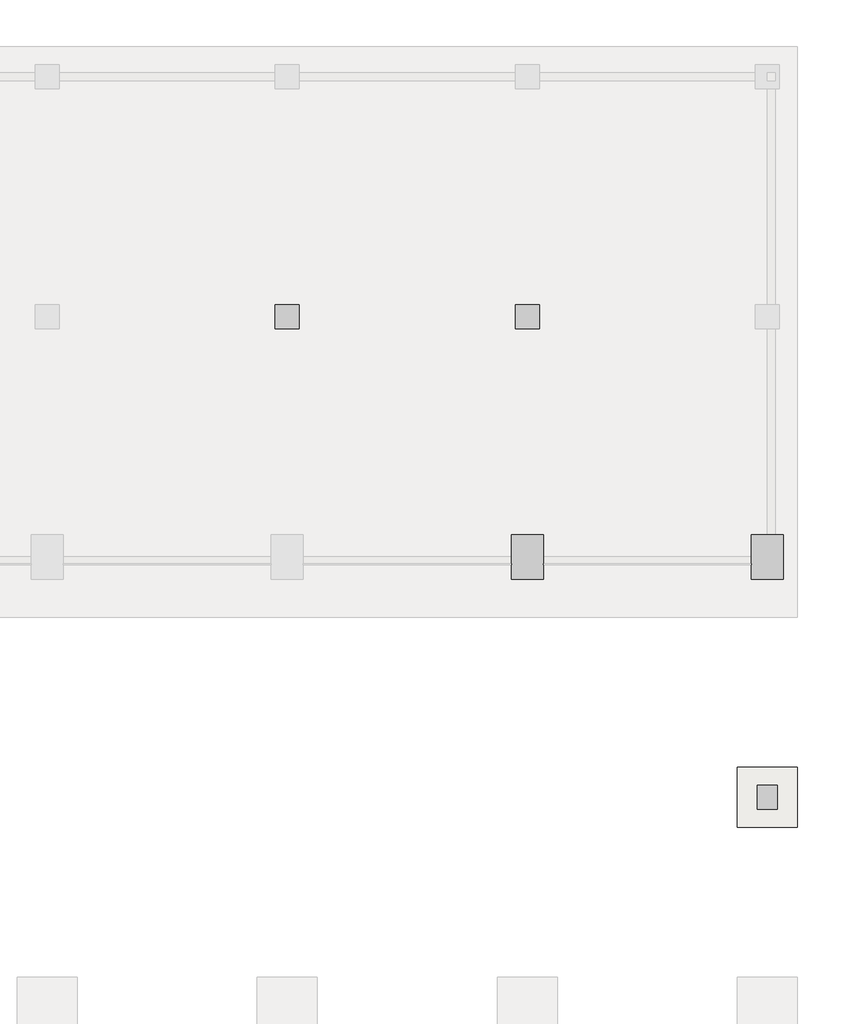
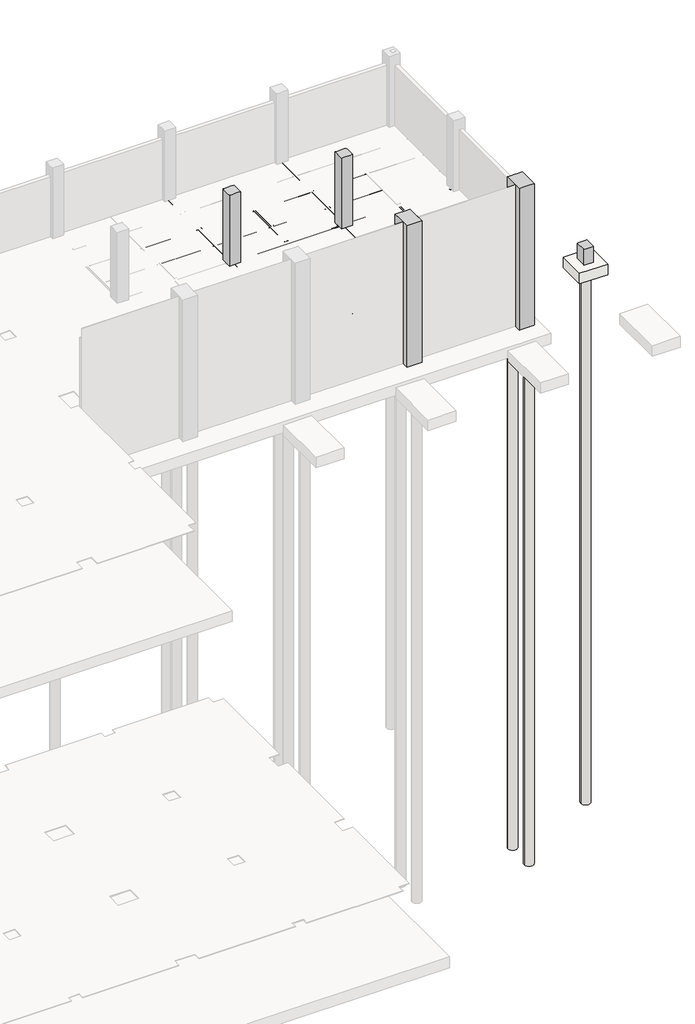
# Not in any storey, part 15 of 16: 29 beams, 5 columns, 4 slabs.
"""IFC4 building model written with IfcOpenShell, lengths in millimetres."""

from ifc_helpers import new_model, si_unit, point, frame, frame_2d, origin, place, context, project, spatial, polyline, circle_curve, trimmed, segment, composite_curve, outline, extrude, faceted_brep, element, save

model = new_model("IFC4")

# Units and contexts
model_context = context("Model", 3, world=origin())
ifc_project = project(units=[si_unit("LENGTHUNIT", "METRE", prefix="MILLI")], contexts=[model_context])

# Site, building
site = spatial("IfcSite", under=ifc_project)
building = spatial("IfcBuilding", under=site)

# Beams
placement = place(None, origin())
element("IfcBeam", 1, ObjectType="Steel Framing_H_KS : H_SB_AR_S02_H-400x200x8x13_BSG2", at=placement, inside=building, context=model_context, shape_type="SweptSolid", body=[
    extrude(outline(composite_curve([segment(polyline([(-4187.0381366, 65900.0), (-4200.0381366, 65900.0), (-4200.0381366, 66100.0), (-4187.0381366, 66100.0), (-4187.0381366, 66020.0)]), True, "CONTINUOUS"), segment(trimmed(circle_curve(frame_2d((-4171.0381366, 66020.0)), 16.0), [point((-4187.0381366, 66020.0))], [point((-4171.0381366, 66004.0))], True, "CARTESIAN"), True, "CONTINUOUS"), segment(polyline([(-4171.0381366, 66004.0), (-3829.0381366, 66004.0)]), True, "CONTINUOUS"), segment(trimmed(circle_curve(frame_2d((-3829.0381366, 66020.0)), 16.0), [point((-3829.0381366, 66004.0))], [point((-3813.0381366, 66020.0))], True, "CARTESIAN"), True, "CONTINUOUS"), segment(polyline([(-3813.0381366, 66020.0), (-3813.0381366, 66100.0), (-3800.0381366, 66100.0), (-3800.0381366, 65900.0), (-3813.0381366, 65900.0), (-3813.0381366, 65980.0)]), True, "CONTINUOUS"), segment(trimmed(circle_curve(frame_2d((-3829.0381366, 65980.0)), 16.0), [point((-3813.0381366, 65980.0))], [point((-3829.0381366, 65996.0))], True, "CARTESIAN"), True, "CONTINUOUS"), segment(polyline([(-3829.0381366, 65996.0), (-4171.0381366, 65996.0)]), True, "CONTINUOUS"), segment(trimmed(circle_curve(frame_2d((-4171.0381366, 65980.0)), 16.0), [point((-4171.0381366, 65996.0))], [point((-4187.0381366, 65980.0))], True, "CARTESIAN"), True, "CONTINUOUS"), segment(polyline([(-4187.0381366, 65980.0), (-4187.0381366, 65900.0)]), True, "CONTINUOUS")], self_intersect=False)), frame((0.0, -11687.3, 0.0), z_axis=(0.0, 1.0, 0.0), x_axis=(0.0, 0.0, 1.0)), (0.0, 0.0, 1.0), 5374.6),
])
element("IfcBeam", 2, ObjectType="Steel Framing_C_KS : H_SB_AR_S02_C-150x75x6.5x10_J1", at=placement, inside=building, context=model_context, shape_type="SweptSolid", body=[
    extrude(outline(composite_curve([segment(polyline([(-8977.2, -3800.0381366), (-8977.2, -3950.0381366), (-9052.2, -3950.0381366)]), True, "CONTINUOUS"), segment(trimmed(circle_curve(frame_2d((-9042.2, -3950.0381366)), 10.0), [point((-9052.2, -3950.0381366))], [point((-9042.2, -3940.0381366))], False, "CARTESIAN"), True, "CONTINUOUS"), segment(polyline([(-9042.2, -3940.0381366), (-8983.7, -3930.7726469), (-8983.7, -3819.3036264), (-9042.2, -3810.0381366)]), True, "CONTINUOUS"), segment(trimmed(circle_curve(frame_2d((-9042.2, -3800.0381366)), 10.0), [point((-9042.2, -3810.0381366))], [point((-9052.2, -3800.0381366))], False, "CARTESIAN"), True, "CONTINUOUS"), segment(polyline([(-9052.2, -3800.0381366), (-8977.2, -3800.0381366)]), True, "CONTINUOUS")], self_intersect=False)), frame((63112.7, 0.0, 0.0), z_axis=(1.0, 0.0, 0.0), x_axis=(0.0, 1.0, 0.0)), (0.0, 0.0, 1.0), 2774.6),
])
element("IfcBeam", 3, ObjectType="Steel Framing_C_KS : H_SB_AR_S02_C-150x75x6.5x10_J1", at=placement, inside=building, context=model_context, shape_type="SweptSolid", body=[
    extrude(outline(composite_curve([segment(polyline([(-10477.2, -3800.0381366), (-10477.2, -3950.0381366), (-10552.2, -3950.0381366)]), True, "CONTINUOUS"), segment(trimmed(circle_curve(frame_2d((-10542.2, -3950.0381366)), 10.0), [point((-10552.2, -3950.0381366))], [point((-10542.2, -3940.0381366))], False, "CARTESIAN"), True, "CONTINUOUS"), segment(polyline([(-10542.2, -3940.0381366), (-10483.7, -3930.7726469), (-10483.7, -3819.3036264), (-10542.2, -3810.0381366)]), True, "CONTINUOUS"), segment(trimmed(circle_curve(frame_2d((-10542.2, -3800.0381366)), 10.0), [point((-10542.2, -3810.0381366))], [point((-10552.2, -3800.0381366))], False, "CARTESIAN"), True, "CONTINUOUS"), segment(polyline([(-10552.2, -3800.0381366), (-10477.2, -3800.0381366)]), True, "CONTINUOUS")], self_intersect=False)), frame((63112.7, 0.0, 0.0), z_axis=(1.0, 0.0, 0.0), x_axis=(0.0, 1.0, 0.0)), (0.0, 0.0, 1.0), 2774.6),
])
element("IfcBeam", 4, ObjectType="Steel Framing_H_KS : H_SB_AR_S02_H-400x200x8x13_BSG1", at=placement, inside=building, context=model_context, shape_type="SweptSolid", body=[
    extrude(outline(composite_curve([segment(polyline([(-11900.0, -4187.0381366), (-11900.0, -4200.0381366), (-12100.0, -4200.0381366), (-12100.0, -4187.0381366), (-12020.0, -4187.0381366)]), True, "CONTINUOUS"), segment(trimmed(circle_curve(frame_2d((-12020.0, -4171.0381366)), 16.0), [point((-12020.0, -4187.0381366))], [point((-12004.0, -4171.0381366))], True, "CARTESIAN"), True, "CONTINUOUS"), segment(polyline([(-12004.0, -4171.0381366), (-12004.0, -3829.0381366)]), True, "CONTINUOUS"), segment(trimmed(circle_curve(frame_2d((-12020.0, -3829.0381366)), 16.0), [point((-12004.0, -3829.0381366))], [point((-12020.0, -3813.0381366))], True, "CARTESIAN"), True, "CONTINUOUS"), segment(polyline([(-12020.0, -3813.0381366), (-12100.0, -3813.0381366), (-12100.0, -3800.0381366), (-11900.0, -3800.0381366), (-11900.0, -3813.0381366), (-11980.0, -3813.0381366)]), True, "CONTINUOUS"), segment(trimmed(circle_curve(frame_2d((-11980.0, -3829.0381366)), 16.0), [point((-11980.0, -3813.0381366))], [point((-11996.0, -3829.0381366))], True, "CARTESIAN"), True, "CONTINUOUS"), segment(polyline([(-11996.0, -3829.0381366), (-11996.0, -4171.0381366)]), True, "CONTINUOUS"), segment(trimmed(circle_curve(frame_2d((-11980.0, -4171.0381366)), 16.0), [point((-11996.0, -4171.0381366))], [point((-11980.0, -4187.0381366))], True, "CARTESIAN"), True, "CONTINUOUS"), segment(polyline([(-11980.0, -4187.0381366), (-11900.0, -4187.0381366)]), True, "CONTINUOUS")], self_intersect=False)), frame((66312.7, 0.0, 0.0), z_axis=(1.0, 0.0, 0.0), x_axis=(0.0, 1.0, 0.0)), (0.0, 0.0, 1.0), 5374.6),
])
element("IfcBeam", 5, ObjectType="Steel Framing_H_KS : H_SB_AR_S02_H-400x200x8x13_BSG2", at=placement, inside=building, context=model_context, shape_type="SweptSolid", body=[
    extrude(outline(composite_curve([segment(polyline([(-4187.0381366, 71900.0), (-4200.0381366, 71900.0), (-4200.0381366, 72100.0), (-4187.0381366, 72100.0), (-4187.0381366, 72020.0)]), True, "CONTINUOUS"), segment(trimmed(circle_curve(frame_2d((-4171.0381366, 72020.0)), 16.0), [point((-4187.0381366, 72020.0))], [point((-4171.0381366, 72004.0))], True, "CARTESIAN"), True, "CONTINUOUS"), segment(polyline([(-4171.0381366, 72004.0), (-3829.0381366, 72004.0)]), True, "CONTINUOUS"), segment(trimmed(circle_curve(frame_2d((-3829.0381366, 72020.0)), 16.0), [point((-3829.0381366, 72004.0))], [point((-3813.0381366, 72020.0))], True, "CARTESIAN"), True, "CONTINUOUS"), segment(polyline([(-3813.0381366, 72020.0), (-3813.0381366, 72100.0), (-3800.0381366, 72100.0), (-3800.0381366, 71900.0), (-3813.0381366, 71900.0), (-3813.0381366, 71980.0)]), True, "CONTINUOUS"), segment(trimmed(circle_curve(frame_2d((-3829.0381366, 71980.0)), 16.0), [point((-3813.0381366, 71980.0))], [point((-3829.0381366, 71996.0))], True, "CARTESIAN"), True, "CONTINUOUS"), segment(polyline([(-3829.0381366, 71996.0), (-4171.0381366, 71996.0)]), True, "CONTINUOUS"), segment(trimmed(circle_curve(frame_2d((-4171.0381366, 71980.0)), 16.0), [point((-4171.0381366, 71996.0))], [point((-4187.0381366, 71980.0))], True, "CARTESIAN"), True, "CONTINUOUS"), segment(polyline([(-4187.0381366, 71980.0), (-4187.0381366, 71900.0)]), True, "CONTINUOUS")], self_intersect=False)), frame((0.0, -11687.3, 0.0), z_axis=(0.0, 1.0, 0.0), x_axis=(0.0, 0.0, 1.0)), (0.0, 0.0, 1.0), 5374.6),
])
element("IfcBeam", 6, ObjectType="Steel Framing_H_KS : H_SB_AR_S02_H-400x200x8x13_BSB1", at=placement, inside=building, context=model_context, shape_type="SweptSolid", body=[
    extrude(outline(composite_curve([segment(polyline([(-4187.0381366, 68900.0), (-4200.0381366, 68900.0), (-4200.0381366, 69100.0), (-4187.0381366, 69100.0), (-4187.0381366, 69020.0)]), True, "CONTINUOUS"), segment(trimmed(circle_curve(frame_2d((-4171.0381366, 69020.0)), 16.0), [point((-4187.0381366, 69020.0))], [point((-4171.0381366, 69004.0))], True, "CARTESIAN"), True, "CONTINUOUS"), segment(polyline([(-4171.0381366, 69004.0), (-3829.0381366, 69004.0)]), True, "CONTINUOUS"), segment(trimmed(circle_curve(frame_2d((-3829.0381366, 69020.0)), 16.0), [point((-3829.0381366, 69004.0))], [point((-3813.0381366, 69020.0))], True, "CARTESIAN"), True, "CONTINUOUS"), segment(polyline([(-3813.0381366, 69020.0), (-3813.0381366, 69100.0), (-3800.0381366, 69100.0), (-3800.0381366, 68900.0), (-3813.0381366, 68900.0), (-3813.0381366, 68980.0)]), True, "CONTINUOUS"), segment(trimmed(circle_curve(frame_2d((-3829.0381366, 68980.0)), 16.0), [point((-3813.0381366, 68980.0))], [point((-3829.0381366, 68996.0))], True, "CARTESIAN"), True, "CONTINUOUS"), segment(polyline([(-3829.0381366, 68996.0), (-4171.0381366, 68996.0)]), True, "CONTINUOUS"), segment(trimmed(circle_curve(frame_2d((-4171.0381366, 68980.0)), 16.0), [point((-4171.0381366, 68996.0))], [point((-4187.0381366, 68980.0))], True, "CARTESIAN"), True, "CONTINUOUS"), segment(polyline([(-4187.0381366, 68980.0), (-4187.0381366, 68900.0)]), True, "CONTINUOUS")], self_intersect=False)), frame((0.0, -11887.3, 0.0), z_axis=(0.0, 1.0, 0.0), x_axis=(0.0, 0.0, 1.0)), (0.0, 0.0, 1.0), 5887.3),
])
element("IfcBeam", 7, ObjectType="Steel Framing_C_KS : H_SB_AR_S02_C-150x75x6.5x10_J1", at=placement, inside=building, context=model_context, shape_type="SweptSolid", body=[
    extrude(outline(composite_curve([segment(polyline([(-8977.2, -3800.0381366), (-8977.2, -3950.0381366), (-9052.2, -3950.0381366)]), True, "CONTINUOUS"), segment(trimmed(circle_curve(frame_2d((-9042.2, -3950.0381366)), 10.0), [point((-9052.2, -3950.0381366))], [point((-9042.2, -3940.0381366))], False, "CARTESIAN"), True, "CONTINUOUS"), segment(polyline([(-9042.2, -3940.0381366), (-8983.7, -3930.7726469), (-8983.7, -3819.3036264), (-9042.2, -3810.0381366)]), True, "CONTINUOUS"), segment(trimmed(circle_curve(frame_2d((-9042.2, -3800.0381366)), 10.0), [point((-9042.2, -3810.0381366))], [point((-9052.2, -3800.0381366))], False, "CARTESIAN"), True, "CONTINUOUS"), segment(polyline([(-9052.2, -3800.0381366), (-8977.2, -3800.0381366)]), True, "CONTINUOUS")], self_intersect=False)), frame((66112.7, 0.0, 0.0), z_axis=(1.0, 0.0, 0.0), x_axis=(0.0, 1.0, 0.0)), (0.0, 0.0, 1.0), 2774.6),
])
element("IfcBeam", 8, ObjectType="Steel Framing_C_KS : H_SB_AR_S02_C-150x75x6.5x10_J1", at=placement, inside=building, context=model_context, shape_type="SweptSolid", body=[
    extrude(outline(composite_curve([segment(polyline([(-10477.2, -3800.0381366), (-10477.2, -3950.0381366), (-10552.2, -3950.0381366)]), True, "CONTINUOUS"), segment(trimmed(circle_curve(frame_2d((-10542.2, -3950.0381366)), 10.0), [point((-10552.2, -3950.0381366))], [point((-10542.2, -3940.0381366))], False, "CARTESIAN"), True, "CONTINUOUS"), segment(polyline([(-10542.2, -3940.0381366), (-10483.7, -3930.7726469), (-10483.7, -3819.3036264), (-10542.2, -3810.0381366)]), True, "CONTINUOUS"), segment(trimmed(circle_curve(frame_2d((-10542.2, -3800.0381366)), 10.0), [point((-10542.2, -3810.0381366))], [point((-10552.2, -3800.0381366))], False, "CARTESIAN"), True, "CONTINUOUS"), segment(polyline([(-10552.2, -3800.0381366), (-10477.2, -3800.0381366)]), True, "CONTINUOUS")], self_intersect=False)), frame((66112.7, 0.0, 0.0), z_axis=(1.0, 0.0, 0.0), x_axis=(0.0, 1.0, 0.0)), (0.0, 0.0, 1.0), 2774.6),
])
element("IfcBeam", 9, ObjectType="Steel Framing_C_KS : H_SB_AR_S02_C-150x75x6.5x10_J1", at=placement, inside=building, context=model_context, shape_type="SweptSolid", body=[
    extrude(outline(composite_curve([segment(polyline([(-8977.2, -3800.0381366), (-8977.2, -3950.0381366), (-9052.2, -3950.0381366)]), True, "CONTINUOUS"), segment(trimmed(circle_curve(frame_2d((-9042.2, -3950.0381366)), 10.0), [point((-9052.2, -3950.0381366))], [point((-9042.2, -3940.0381366))], False, "CARTESIAN"), True, "CONTINUOUS"), segment(polyline([(-9042.2, -3940.0381366), (-8983.7, -3930.7726469), (-8983.7, -3819.3036264), (-9042.2, -3810.0381366)]), True, "CONTINUOUS"), segment(trimmed(circle_curve(frame_2d((-9042.2, -3800.0381366)), 10.0), [point((-9042.2, -3810.0381366))], [point((-9052.2, -3800.0381366))], False, "CARTESIAN"), True, "CONTINUOUS"), segment(polyline([(-9052.2, -3800.0381366), (-8977.2, -3800.0381366)]), True, "CONTINUOUS")], self_intersect=False)), frame((69112.7, 0.0, 0.0), z_axis=(1.0, 0.0, 0.0), x_axis=(0.0, 1.0, 0.0)), (0.0, 0.0, 1.0), 2774.6),
])
element("IfcBeam", 10, ObjectType="Steel Framing_C_KS : H_SB_AR_S02_C-150x75x6.5x10_J1", at=placement, inside=building, context=model_context, shape_type="SweptSolid", body=[
    extrude(outline(composite_curve([segment(polyline([(-10477.2, -3800.0381366), (-10477.2, -3950.0381366), (-10552.2, -3950.0381366)]), True, "CONTINUOUS"), segment(trimmed(circle_curve(frame_2d((-10542.2, -3950.0381366)), 10.0), [point((-10552.2, -3950.0381366))], [point((-10542.2, -3940.0381366))], False, "CARTESIAN"), True, "CONTINUOUS"), segment(polyline([(-10542.2, -3940.0381366), (-10483.7, -3930.7726469), (-10483.7, -3819.3036264), (-10542.2, -3810.0381366)]), True, "CONTINUOUS"), segment(trimmed(circle_curve(frame_2d((-10542.2, -3800.0381366)), 10.0), [point((-10542.2, -3810.0381366))], [point((-10552.2, -3800.0381366))], False, "CARTESIAN"), True, "CONTINUOUS"), segment(polyline([(-10552.2, -3800.0381366), (-10477.2, -3800.0381366)]), True, "CONTINUOUS")], self_intersect=False)), frame((69112.7, 0.0, 0.0), z_axis=(1.0, 0.0, 0.0), x_axis=(0.0, 1.0, 0.0)), (0.0, 0.0, 1.0), 2774.6),
])
element("IfcBeam", 11, ObjectType="Steel Framing_H_KS : H_SB_AR_S02_H-400x200x8x13_BSG1", at=placement, inside=building, context=model_context, shape_type="SweptSolid", body=[
    extrude(outline(composite_curve([segment(polyline([(-11900.0, -4187.0381366), (-11900.0, -4200.0381366), (-12100.0, -4200.0381366), (-12100.0, -4187.0381366), (-12020.0, -4187.0381366)]), True, "CONTINUOUS"), segment(trimmed(circle_curve(frame_2d((-12020.0, -4171.0381366)), 16.0), [point((-12020.0, -4187.0381366))], [point((-12004.0, -4171.0381366))], True, "CARTESIAN"), True, "CONTINUOUS"), segment(polyline([(-12004.0, -4171.0381366), (-12004.0, -3829.0381366)]), True, "CONTINUOUS"), segment(trimmed(circle_curve(frame_2d((-12020.0, -3829.0381366)), 16.0), [point((-12004.0, -3829.0381366))], [point((-12020.0, -3813.0381366))], True, "CARTESIAN"), True, "CONTINUOUS"), segment(polyline([(-12020.0, -3813.0381366), (-12100.0, -3813.0381366), (-12100.0, -3800.0381366), (-11900.0, -3800.0381366), (-11900.0, -3813.0381366), (-11980.0, -3813.0381366)]), True, "CONTINUOUS"), segment(trimmed(circle_curve(frame_2d((-11980.0, -3829.0381366)), 16.0), [point((-11980.0, -3813.0381366))], [point((-11996.0, -3829.0381366))], True, "CARTESIAN"), True, "CONTINUOUS"), segment(polyline([(-11996.0, -3829.0381366), (-11996.0, -4171.0381366)]), True, "CONTINUOUS"), segment(trimmed(circle_curve(frame_2d((-11980.0, -4171.0381366)), 16.0), [point((-11996.0, -4171.0381366))], [point((-11980.0, -4187.0381366))], True, "CARTESIAN"), True, "CONTINUOUS"), segment(polyline([(-11980.0, -4187.0381366), (-11900.0, -4187.0381366)]), True, "CONTINUOUS")], self_intersect=False)), frame((72312.7, 0.0, 0.0), z_axis=(1.0, 0.0, 0.0), x_axis=(0.0, 1.0, 0.0)), (0.0, 0.0, 1.0), 5374.6),
])
element("IfcBeam", 12, ObjectType="Steel Framing_C_KS : H_SB_AR_S02_C-150x75x6.5x10_J1", at=placement, inside=building, context=model_context, shape_type="SweptSolid", body=[
    extrude(outline(composite_curve([segment(polyline([(-8977.2, -3800.0381366), (-8977.2, -3950.0381366), (-9052.2, -3950.0381366)]), True, "CONTINUOUS"), segment(trimmed(circle_curve(frame_2d((-9042.2, -3950.0381366)), 10.0), [point((-9052.2, -3950.0381366))], [point((-9042.2, -3940.0381366))], False, "CARTESIAN"), True, "CONTINUOUS"), segment(polyline([(-9042.2, -3940.0381366), (-8983.7, -3930.7726469), (-8983.7, -3819.3036264), (-9042.2, -3810.0381366)]), True, "CONTINUOUS"), segment(trimmed(circle_curve(frame_2d((-9042.2, -3800.0381366)), 10.0), [point((-9042.2, -3810.0381366))], [point((-9052.2, -3800.0381366))], False, "CARTESIAN"), True, "CONTINUOUS"), segment(polyline([(-9052.2, -3800.0381366), (-8977.2, -3800.0381366)]), True, "CONTINUOUS")], self_intersect=False)), frame((72112.7, 0.0, 0.0), z_axis=(1.0, 0.0, 0.0), x_axis=(0.0, 1.0, 0.0)), (0.0, 0.0, 1.0), 2774.6),
])
element("IfcBeam", 13, ObjectType="Steel Framing_C_KS : H_SB_AR_S02_C-150x75x6.5x10_J1", at=placement, inside=building, context=model_context, shape_type="SweptSolid", body=[
    extrude(outline(composite_curve([segment(polyline([(-10477.2, -3800.0381366), (-10477.2, -3950.0381366), (-10552.2, -3950.0381366)]), True, "CONTINUOUS"), segment(trimmed(circle_curve(frame_2d((-10542.2, -3950.0381366)), 10.0), [point((-10552.2, -3950.0381366))], [point((-10542.2, -3940.0381366))], False, "CARTESIAN"), True, "CONTINUOUS"), segment(polyline([(-10542.2, -3940.0381366), (-10483.7, -3930.7726469), (-10483.7, -3819.3036264), (-10542.2, -3810.0381366)]), True, "CONTINUOUS"), segment(trimmed(circle_curve(frame_2d((-10542.2, -3800.0381366)), 10.0), [point((-10542.2, -3810.0381366))], [point((-10552.2, -3800.0381366))], False, "CARTESIAN"), True, "CONTINUOUS"), segment(polyline([(-10552.2, -3800.0381366), (-10477.2, -3800.0381366)]), True, "CONTINUOUS")], self_intersect=False)), frame((72112.7, 0.0, 0.0), z_axis=(1.0, 0.0, 0.0), x_axis=(0.0, 1.0, 0.0)), (0.0, 0.0, 1.0), 2774.6),
])
element("IfcBeam", 14, ObjectType="Steel Framing_H_KS : H_SB_AR_S02_H-400x200x8x13_BSG2", at=placement, inside=building, context=model_context, shape_type="SweptSolid", body=[
    extrude(outline(composite_curve([segment(polyline([(-4187.0381366, 65900.0), (-4200.0381366, 65900.0), (-4200.0381366, 66100.0), (-4187.0381366, 66100.0), (-4187.0381366, 66020.0)]), True, "CONTINUOUS"), segment(trimmed(circle_curve(frame_2d((-4171.0381366, 66020.0)), 16.0), [point((-4187.0381366, 66020.0))], [point((-4171.0381366, 66004.0))], True, "CARTESIAN"), True, "CONTINUOUS"), segment(polyline([(-4171.0381366, 66004.0), (-3829.0381366, 66004.0)]), True, "CONTINUOUS"), segment(trimmed(circle_curve(frame_2d((-3829.0381366, 66020.0)), 16.0), [point((-3829.0381366, 66004.0))], [point((-3813.0381366, 66020.0))], True, "CARTESIAN"), True, "CONTINUOUS"), segment(polyline([(-3813.0381366, 66020.0), (-3813.0381366, 66100.0), (-3800.0381366, 66100.0), (-3800.0381366, 65900.0), (-3813.0381366, 65900.0), (-3813.0381366, 65980.0)]), True, "CONTINUOUS"), segment(trimmed(circle_curve(frame_2d((-3829.0381366, 65980.0)), 16.0), [point((-3813.0381366, 65980.0))], [point((-3829.0381366, 65996.0))], True, "CARTESIAN"), True, "CONTINUOUS"), segment(polyline([(-3829.0381366, 65996.0), (-4171.0381366, 65996.0)]), True, "CONTINUOUS"), segment(trimmed(circle_curve(frame_2d((-4171.0381366, 65980.0)), 16.0), [point((-4171.0381366, 65996.0))], [point((-4187.0381366, 65980.0))], True, "CARTESIAN"), True, "CONTINUOUS"), segment(polyline([(-4187.0381366, 65980.0), (-4187.0381366, 65900.0)]), True, "CONTINUOUS")], self_intersect=False)), frame((0.0, -17437.3, 0.0), z_axis=(0.0, 1.0, 0.0), x_axis=(0.0, 0.0, 1.0)), (0.0, 0.0, 1.0), 5124.6),
])
element("IfcBeam", 15, ObjectType="Steel Framing_C_KS : H_SB_AR_S02_C-150x75x6.5x10_J1", at=placement, inside=building, context=model_context, shape_type="SweptSolid", body=[
    extrude(outline(composite_curve([segment(polyline([(-14977.2, -3800.0381366), (-14977.2, -3950.0381366), (-15052.2, -3950.0381366)]), True, "CONTINUOUS"), segment(trimmed(circle_curve(frame_2d((-15042.2, -3950.0381366)), 10.0), [point((-15052.2, -3950.0381366))], [point((-15042.2, -3940.0381366))], False, "CARTESIAN"), True, "CONTINUOUS"), segment(polyline([(-15042.2, -3940.0381366), (-14983.7, -3930.7726469), (-14983.7, -3819.3036264), (-15042.2, -3810.0381366)]), True, "CONTINUOUS"), segment(trimmed(circle_curve(frame_2d((-15042.2, -3800.0381366)), 10.0), [point((-15042.2, -3810.0381366))], [point((-15052.2, -3800.0381366))], False, "CARTESIAN"), True, "CONTINUOUS"), segment(polyline([(-15052.2, -3800.0381366), (-14977.2, -3800.0381366)]), True, "CONTINUOUS")], self_intersect=False)), frame((63112.7, 0.0, 0.0), z_axis=(1.0, 0.0, 0.0), x_axis=(0.0, 1.0, 0.0)), (0.0, 0.0, 1.0), 2774.6),
])
element("IfcBeam", 16, ObjectType="Steel Framing_C_KS : H_SB_AR_S02_C-150x75x6.5x10_J1", at=placement, inside=building, context=model_context, shape_type="SweptSolid", body=[
    extrude(outline(composite_curve([segment(polyline([(-13477.2, -3800.0381366), (-13477.2, -3950.0381366), (-13552.2, -3950.0381366)]), True, "CONTINUOUS"), segment(trimmed(circle_curve(frame_2d((-13542.2, -3950.0381366)), 10.0), [point((-13552.2, -3950.0381366))], [point((-13542.2, -3940.0381366))], False, "CARTESIAN"), True, "CONTINUOUS"), segment(polyline([(-13542.2, -3940.0381366), (-13483.7, -3930.7726469), (-13483.7, -3819.3036264), (-13542.2, -3810.0381366)]), True, "CONTINUOUS"), segment(trimmed(circle_curve(frame_2d((-13542.2, -3800.0381366)), 10.0), [point((-13542.2, -3810.0381366))], [point((-13552.2, -3800.0381366))], False, "CARTESIAN"), True, "CONTINUOUS"), segment(polyline([(-13552.2, -3800.0381366), (-13477.2, -3800.0381366)]), True, "CONTINUOUS")], self_intersect=False)), frame((63112.7, 0.0, 0.0), z_axis=(1.0, 0.0, 0.0), x_axis=(0.0, 1.0, 0.0)), (0.0, 0.0, 1.0), 2774.6),
])
element("IfcBeam", 17, ObjectType="Steel Framing_H_KS : H_SB_AR_S02_H-400x200x8x13_BSG2", at=placement, inside=building, context=model_context, shape_type="SweptSolid", body=[
    extrude(outline(composite_curve([segment(polyline([(-4187.0381366, 71900.0), (-4200.0381366, 71900.0), (-4200.0381366, 72100.0), (-4187.0381366, 72100.0), (-4187.0381366, 72020.0)]), True, "CONTINUOUS"), segment(trimmed(circle_curve(frame_2d((-4171.0381366, 72020.0)), 16.0), [point((-4187.0381366, 72020.0))], [point((-4171.0381366, 72004.0))], True, "CARTESIAN"), True, "CONTINUOUS"), segment(polyline([(-4171.0381366, 72004.0), (-3829.0381366, 72004.0)]), True, "CONTINUOUS"), segment(trimmed(circle_curve(frame_2d((-3829.0381366, 72020.0)), 16.0), [point((-3829.0381366, 72004.0))], [point((-3813.0381366, 72020.0))], True, "CARTESIAN"), True, "CONTINUOUS"), segment(polyline([(-3813.0381366, 72020.0), (-3813.0381366, 72100.0), (-3800.0381366, 72100.0), (-3800.0381366, 71900.0), (-3813.0381366, 71900.0), (-3813.0381366, 71980.0)]), True, "CONTINUOUS"), segment(trimmed(circle_curve(frame_2d((-3829.0381366, 71980.0)), 16.0), [point((-3813.0381366, 71980.0))], [point((-3829.0381366, 71996.0))], True, "CARTESIAN"), True, "CONTINUOUS"), segment(polyline([(-3829.0381366, 71996.0), (-4171.0381366, 71996.0)]), True, "CONTINUOUS"), segment(trimmed(circle_curve(frame_2d((-4171.0381366, 71980.0)), 16.0), [point((-4171.0381366, 71996.0))], [point((-4187.0381366, 71980.0))], True, "CARTESIAN"), True, "CONTINUOUS"), segment(polyline([(-4187.0381366, 71980.0), (-4187.0381366, 71900.0)]), True, "CONTINUOUS")], self_intersect=False)), frame((0.0, -17437.3, 0.0), z_axis=(0.0, 1.0, 0.0), x_axis=(0.0, 0.0, 1.0)), (0.0, 0.0, 1.0), 5124.6),
])
element("IfcBeam", 18, ObjectType="Steel Framing_H_KS : H_SB_AR_S02_H-400x200x8x13_BSB1", at=placement, inside=building, context=model_context, shape_type="SweptSolid", body=[
    extrude(outline(composite_curve([segment(polyline([(-4187.0381366, 68900.0), (-4200.0381366, 68900.0), (-4200.0381366, 69100.0), (-4187.0381366, 69100.0), (-4187.0381366, 69020.0)]), True, "CONTINUOUS"), segment(trimmed(circle_curve(frame_2d((-4171.0381366, 69020.0)), 16.0), [point((-4187.0381366, 69020.0))], [point((-4171.0381366, 69004.0))], True, "CARTESIAN"), True, "CONTINUOUS"), segment(polyline([(-4171.0381366, 69004.0), (-3829.0381366, 69004.0)]), True, "CONTINUOUS"), segment(trimmed(circle_curve(frame_2d((-3829.0381366, 69020.0)), 16.0), [point((-3829.0381366, 69004.0))], [point((-3813.0381366, 69020.0))], True, "CARTESIAN"), True, "CONTINUOUS"), segment(polyline([(-3813.0381366, 69020.0), (-3813.0381366, 69100.0), (-3800.0381366, 69100.0), (-3800.0381366, 68900.0), (-3813.0381366, 68900.0), (-3813.0381366, 68980.0)]), True, "CONTINUOUS"), segment(trimmed(circle_curve(frame_2d((-3829.0381366, 68980.0)), 16.0), [point((-3813.0381366, 68980.0))], [point((-3829.0381366, 68996.0))], True, "CARTESIAN"), True, "CONTINUOUS"), segment(polyline([(-3829.0381366, 68996.0), (-4171.0381366, 68996.0)]), True, "CONTINUOUS"), segment(trimmed(circle_curve(frame_2d((-4171.0381366, 68980.0)), 16.0), [point((-4171.0381366, 68996.0))], [point((-4187.0381366, 68980.0))], True, "CARTESIAN"), True, "CONTINUOUS"), segment(polyline([(-4187.0381366, 68980.0), (-4187.0381366, 68900.0)]), True, "CONTINUOUS")], self_intersect=False)), frame((0.0, -18000.0, 0.0), z_axis=(0.0, 1.0, 0.0), x_axis=(0.0, 0.0, 1.0)), (0.0, 0.0, 1.0), 5887.3),
])
element("IfcBeam", 19, ObjectType="Steel Framing_C_KS : H_SB_AR_S02_C-150x75x6.5x10_J1", at=placement, inside=building, context=model_context, shape_type="SweptSolid", body=[
    extrude(outline(composite_curve([segment(polyline([(-14977.2, -3800.0381366), (-14977.2, -3950.0381366), (-15052.2, -3950.0381366)]), True, "CONTINUOUS"), segment(trimmed(circle_curve(frame_2d((-15042.2, -3950.0381366)), 10.0), [point((-15052.2, -3950.0381366))], [point((-15042.2, -3940.0381366))], False, "CARTESIAN"), True, "CONTINUOUS"), segment(polyline([(-15042.2, -3940.0381366), (-14983.7, -3930.7726469), (-14983.7, -3819.3036264), (-15042.2, -3810.0381366)]), True, "CONTINUOUS"), segment(trimmed(circle_curve(frame_2d((-15042.2, -3800.0381366)), 10.0), [point((-15042.2, -3810.0381366))], [point((-15052.2, -3800.0381366))], False, "CARTESIAN"), True, "CONTINUOUS"), segment(polyline([(-15052.2, -3800.0381366), (-14977.2, -3800.0381366)]), True, "CONTINUOUS")], self_intersect=False)), frame((66112.7, 0.0, 0.0), z_axis=(1.0, 0.0, 0.0), x_axis=(0.0, 1.0, 0.0)), (0.0, 0.0, 1.0), 2774.6),
])
element("IfcBeam", 20, ObjectType="Steel Framing_C_KS : H_SB_AR_S02_C-150x75x6.5x10_J1", at=placement, inside=building, context=model_context, shape_type="SweptSolid", body=[
    extrude(outline(composite_curve([segment(polyline([(-13477.2, -3800.0381366), (-13477.2, -3950.0381366), (-13552.2, -3950.0381366)]), True, "CONTINUOUS"), segment(trimmed(circle_curve(frame_2d((-13542.2, -3950.0381366)), 10.0), [point((-13552.2, -3950.0381366))], [point((-13542.2, -3940.0381366))], False, "CARTESIAN"), True, "CONTINUOUS"), segment(polyline([(-13542.2, -3940.0381366), (-13483.7, -3930.7726469), (-13483.7, -3819.3036264), (-13542.2, -3810.0381366)]), True, "CONTINUOUS"), segment(trimmed(circle_curve(frame_2d((-13542.2, -3800.0381366)), 10.0), [point((-13542.2, -3810.0381366))], [point((-13552.2, -3800.0381366))], False, "CARTESIAN"), True, "CONTINUOUS"), segment(polyline([(-13552.2, -3800.0381366), (-13477.2, -3800.0381366)]), True, "CONTINUOUS")], self_intersect=False)), frame((66112.7, 0.0, 0.0), z_axis=(1.0, 0.0, 0.0), x_axis=(0.0, 1.0, 0.0)), (0.0, 0.0, 1.0), 2774.6),
])
element("IfcBeam", 21, ObjectType="Steel Framing_C_KS : H_SB_AR_S02_C-150x75x6.5x10_J1", at=placement, inside=building, context=model_context, shape_type="SweptSolid", body=[
    extrude(outline(composite_curve([segment(polyline([(-14977.2, -3800.0381366), (-14977.2, -3950.0381366), (-15052.2, -3950.0381366)]), True, "CONTINUOUS"), segment(trimmed(circle_curve(frame_2d((-15042.2, -3950.0381366)), 10.0), [point((-15052.2, -3950.0381366))], [point((-15042.2, -3940.0381366))], False, "CARTESIAN"), True, "CONTINUOUS"), segment(polyline([(-15042.2, -3940.0381366), (-14983.7, -3930.7726469), (-14983.7, -3819.3036264), (-15042.2, -3810.0381366)]), True, "CONTINUOUS"), segment(trimmed(circle_curve(frame_2d((-15042.2, -3800.0381366)), 10.0), [point((-15042.2, -3810.0381366))], [point((-15052.2, -3800.0381366))], False, "CARTESIAN"), True, "CONTINUOUS"), segment(polyline([(-15052.2, -3800.0381366), (-14977.2, -3800.0381366)]), True, "CONTINUOUS")], self_intersect=False)), frame((69112.7, 0.0, 0.0), z_axis=(1.0, 0.0, 0.0), x_axis=(0.0, 1.0, 0.0)), (0.0, 0.0, 1.0), 2774.6),
])
element("IfcBeam", 22, ObjectType="Steel Framing_C_KS : H_SB_AR_S02_C-150x75x6.5x10_J1", at=placement, inside=building, context=model_context, shape_type="SweptSolid", body=[
    extrude(outline(composite_curve([segment(polyline([(-13477.2, -3800.0381366), (-13477.2, -3950.0381366), (-13552.2, -3950.0381366)]), True, "CONTINUOUS"), segment(trimmed(circle_curve(frame_2d((-13542.2, -3950.0381366)), 10.0), [point((-13552.2, -3950.0381366))], [point((-13542.2, -3940.0381366))], False, "CARTESIAN"), True, "CONTINUOUS"), segment(polyline([(-13542.2, -3940.0381366), (-13483.7, -3930.7726469), (-13483.7, -3819.3036264), (-13542.2, -3810.0381366)]), True, "CONTINUOUS"), segment(trimmed(circle_curve(frame_2d((-13542.2, -3800.0381366)), 10.0), [point((-13542.2, -3810.0381366))], [point((-13552.2, -3800.0381366))], False, "CARTESIAN"), True, "CONTINUOUS"), segment(polyline([(-13552.2, -3800.0381366), (-13477.2, -3800.0381366)]), True, "CONTINUOUS")], self_intersect=False)), frame((69112.7, 0.0, 0.0), z_axis=(1.0, 0.0, 0.0), x_axis=(0.0, 1.0, 0.0)), (0.0, 0.0, 1.0), 2774.6),
])
element("IfcBeam", 23, ObjectType="Steel Framing_H_KS : H_SB_AR_S02_H-400x200x8x13_BSB1", at=placement, inside=building, context=model_context, shape_type="SweptSolid", body=[
    extrude(outline(composite_curve([segment(polyline([(-4187.0381366, 74900.0), (-4200.0381366, 74900.0), (-4200.0381366, 75100.0), (-4187.0381366, 75100.0), (-4187.0381366, 75020.0)]), True, "CONTINUOUS"), segment(trimmed(circle_curve(frame_2d((-4171.0381366, 75020.0)), 16.0), [point((-4187.0381366, 75020.0))], [point((-4171.0381366, 75004.0))], True, "CARTESIAN"), True, "CONTINUOUS"), segment(polyline([(-4171.0381366, 75004.0), (-3829.0381366, 75004.0)]), True, "CONTINUOUS"), segment(trimmed(circle_curve(frame_2d((-3829.0381366, 75020.0)), 16.0), [point((-3829.0381366, 75004.0))], [point((-3813.0381366, 75020.0))], True, "CARTESIAN"), True, "CONTINUOUS"), segment(polyline([(-3813.0381366, 75020.0), (-3813.0381366, 75100.0), (-3800.0381366, 75100.0), (-3800.0381366, 74900.0), (-3813.0381366, 74900.0), (-3813.0381366, 74980.0)]), True, "CONTINUOUS"), segment(trimmed(circle_curve(frame_2d((-3829.0381366, 74980.0)), 16.0), [point((-3813.0381366, 74980.0))], [point((-3829.0381366, 74996.0))], True, "CARTESIAN"), True, "CONTINUOUS"), segment(polyline([(-3829.0381366, 74996.0), (-4171.0381366, 74996.0)]), True, "CONTINUOUS"), segment(trimmed(circle_curve(frame_2d((-4171.0381366, 74980.0)), 16.0), [point((-4171.0381366, 74996.0))], [point((-4187.0381366, 74980.0))], True, "CARTESIAN"), True, "CONTINUOUS"), segment(polyline([(-4187.0381366, 74980.0), (-4187.0381366, 74900.0)]), True, "CONTINUOUS")], self_intersect=False)), frame((0.0, -18000.0, 0.0), z_axis=(0.0, 1.0, 0.0), x_axis=(0.0, 0.0, 1.0)), (0.0, 0.0, 1.0), 5887.3),
])
element("IfcBeam", 24, ObjectType="Steel Framing_C_KS : H_SB_AR_S02_C-150x75x6.5x10_J1", at=placement, inside=building, context=model_context, shape_type="SweptSolid", body=[
    extrude(outline(composite_curve([segment(polyline([(-14977.2, -3800.0381366), (-14977.2, -3950.0381366), (-15052.2, -3950.0381366)]), True, "CONTINUOUS"), segment(trimmed(circle_curve(frame_2d((-15042.2, -3950.0381366)), 10.0), [point((-15052.2, -3950.0381366))], [point((-15042.2, -3940.0381366))], False, "CARTESIAN"), True, "CONTINUOUS"), segment(polyline([(-15042.2, -3940.0381366), (-14983.7, -3930.7726469), (-14983.7, -3819.3036264), (-15042.2, -3810.0381366)]), True, "CONTINUOUS"), segment(trimmed(circle_curve(frame_2d((-15042.2, -3800.0381366)), 10.0), [point((-15042.2, -3810.0381366))], [point((-15052.2, -3800.0381366))], False, "CARTESIAN"), True, "CONTINUOUS"), segment(polyline([(-15052.2, -3800.0381366), (-14977.2, -3800.0381366)]), True, "CONTINUOUS")], self_intersect=False)), frame((72112.7, 0.0, 0.0), z_axis=(1.0, 0.0, 0.0), x_axis=(0.0, 1.0, 0.0)), (0.0, 0.0, 1.0), 2774.6),
])
element("IfcBeam", 25, ObjectType="Steel Framing_C_KS : H_SB_AR_S02_C-150x75x6.5x10_J1", at=placement, inside=building, context=model_context, shape_type="SweptSolid", body=[
    extrude(outline(composite_curve([segment(polyline([(-16477.2, -3800.0381366), (-16477.2, -3950.0381366), (-16552.2, -3950.0381366)]), True, "CONTINUOUS"), segment(trimmed(circle_curve(frame_2d((-16542.2, -3950.0381366)), 10.0), [point((-16552.2, -3950.0381366))], [point((-16542.2, -3940.0381366))], False, "CARTESIAN"), True, "CONTINUOUS"), segment(polyline([(-16542.2, -3940.0381366), (-16483.7, -3930.7726469), (-16483.7, -3819.3036264), (-16542.2, -3810.0381366)]), True, "CONTINUOUS"), segment(trimmed(circle_curve(frame_2d((-16542.2, -3800.0381366)), 10.0), [point((-16542.2, -3810.0381366))], [point((-16552.2, -3800.0381366))], False, "CARTESIAN"), True, "CONTINUOUS"), segment(polyline([(-16552.2, -3800.0381366), (-16477.2, -3800.0381366)]), True, "CONTINUOUS")], self_intersect=False)), frame((72112.7, 0.0, 0.0), z_axis=(1.0, 0.0, 0.0), x_axis=(0.0, 1.0, 0.0)), (0.0, 0.0, 1.0), 2774.6),
])
element("IfcBeam", 26, ObjectType="Steel Framing_C_KS : H_SB_AR_S02_C-150x75x6.5x10_J1", at=placement, inside=building, context=model_context, shape_type="SweptSolid", body=[
    extrude(outline(composite_curve([segment(polyline([(-13477.2, -3800.0381366), (-13477.2, -3950.0381366), (-13552.2, -3950.0381366)]), True, "CONTINUOUS"), segment(trimmed(circle_curve(frame_2d((-13542.2, -3950.0381366)), 10.0), [point((-13552.2, -3950.0381366))], [point((-13542.2, -3940.0381366))], False, "CARTESIAN"), True, "CONTINUOUS"), segment(polyline([(-13542.2, -3940.0381366), (-13483.7, -3930.7726469), (-13483.7, -3819.3036264), (-13542.2, -3810.0381366)]), True, "CONTINUOUS"), segment(trimmed(circle_curve(frame_2d((-13542.2, -3800.0381366)), 10.0), [point((-13542.2, -3810.0381366))], [point((-13552.2, -3800.0381366))], False, "CARTESIAN"), True, "CONTINUOUS"), segment(polyline([(-13552.2, -3800.0381366), (-13477.2, -3800.0381366)]), True, "CONTINUOUS")], self_intersect=False)), frame((72112.7, 0.0, 0.0), z_axis=(1.0, 0.0, 0.0), x_axis=(0.0, 1.0, 0.0)), (0.0, 0.0, 1.0), 2774.6),
])
element("IfcBeam", 27, ObjectType="Steel Framing_C_KS : H_SB_AR_S02_C-150x75x6.5x10_J1", at=placement, inside=building, context=model_context, shape_type="SweptSolid", body=[
    extrude(outline(composite_curve([segment(polyline([(-14977.2, -3800.0381366), (-14977.2, -3950.0381366), (-15052.2, -3950.0381366)]), True, "CONTINUOUS"), segment(trimmed(circle_curve(frame_2d((-15042.2, -3950.0381366)), 10.0), [point((-15052.2, -3950.0381366))], [point((-15042.2, -3940.0381366))], False, "CARTESIAN"), True, "CONTINUOUS"), segment(polyline([(-15042.2, -3940.0381366), (-14983.7, -3930.7726469), (-14983.7, -3819.3036264), (-15042.2, -3810.0381366)]), True, "CONTINUOUS"), segment(trimmed(circle_curve(frame_2d((-15042.2, -3800.0381366)), 10.0), [point((-15042.2, -3810.0381366))], [point((-15052.2, -3800.0381366))], False, "CARTESIAN"), True, "CONTINUOUS"), segment(polyline([(-15052.2, -3800.0381366), (-14977.2, -3800.0381366)]), True, "CONTINUOUS")], self_intersect=False)), frame((75112.7, 0.0, 0.0), z_axis=(1.0, 0.0, 0.0), x_axis=(0.0, 1.0, 0.0)), (0.0, 0.0, 1.0), 2887.3),
])
element("IfcBeam", 28, ObjectType="Steel Framing_C_KS : H_SB_AR_S02_C-150x75x6.5x10_J1", at=placement, inside=building, context=model_context, shape_type="SweptSolid", body=[
    extrude(outline(composite_curve([segment(polyline([(-16477.2, -3800.0381366), (-16477.2, -3950.0381366), (-16552.2, -3950.0381366)]), True, "CONTINUOUS"), segment(trimmed(circle_curve(frame_2d((-16542.2, -3950.0381366)), 10.0), [point((-16552.2, -3950.0381366))], [point((-16542.2, -3940.0381366))], False, "CARTESIAN"), True, "CONTINUOUS"), segment(polyline([(-16542.2, -3940.0381366), (-16483.7, -3930.7726469), (-16483.7, -3819.3036264), (-16542.2, -3810.0381366)]), True, "CONTINUOUS"), segment(trimmed(circle_curve(frame_2d((-16542.2, -3800.0381366)), 10.0), [point((-16542.2, -3810.0381366))], [point((-16552.2, -3800.0381366))], False, "CARTESIAN"), True, "CONTINUOUS"), segment(polyline([(-16552.2, -3800.0381366), (-16477.2, -3800.0381366)]), True, "CONTINUOUS")], self_intersect=False)), frame((75112.7, 0.0, 0.0), z_axis=(1.0, 0.0, 0.0), x_axis=(0.0, 1.0, 0.0)), (0.0, 0.0, 1.0), 2887.3),
])
element("IfcBeam", 29, ObjectType="Steel Framing_C_KS : H_SB_AR_S02_C-150x75x6.5x10_J1", at=placement, inside=building, context=model_context, shape_type="SweptSolid", body=[
    extrude(outline(composite_curve([segment(polyline([(-13477.2, -3800.0381366), (-13477.2, -3950.0381366), (-13552.2, -3950.0381366)]), True, "CONTINUOUS"), segment(trimmed(circle_curve(frame_2d((-13542.2, -3950.0381366)), 10.0), [point((-13552.2, -3950.0381366))], [point((-13542.2, -3940.0381366))], False, "CARTESIAN"), True, "CONTINUOUS"), segment(polyline([(-13542.2, -3940.0381366), (-13483.7, -3930.7726469), (-13483.7, -3819.3036264), (-13542.2, -3810.0381366)]), True, "CONTINUOUS"), segment(trimmed(circle_curve(frame_2d((-13542.2, -3800.0381366)), 10.0), [point((-13542.2, -3810.0381366))], [point((-13552.2, -3800.0381366))], False, "CARTESIAN"), True, "CONTINUOUS"), segment(polyline([(-13552.2, -3800.0381366), (-13477.2, -3800.0381366)]), True, "CONTINUOUS")], self_intersect=False)), frame((75112.7, 0.0, 0.0), z_axis=(1.0, 0.0, 0.0), x_axis=(0.0, 1.0, 0.0)), (0.0, 0.0, 1.0), 2887.3),
])

# Columns
element("IfcColumn", 30, ObjectType="RC_Column_Rectangular : H_SC_AR_S15_UG PED_Bit_800x1100_PD1", at=placement, inside=building, context=model_context, shape_type="Brep", body=[
    faceted_brep([(72400.0, -17450.0, -7800.0381366), (72400.0, -18000.0, -7800.0381366), (72400.0, -18200.0, -7800.0381366), (72400.0, -18550.0, -7800.0381366), (71600.0, -18550.0, -7800.0381366), (71600.0, -18200.0, -7800.0381366), (71600.0, -18000.0, -7800.0381366), (71600.0, -17450.0, -7800.0381366), (72400.0, -17450.0, 199.9618634), (72400.0, -17825.0, 199.9618634), (72400.0, -18000.0, 199.9618634), (72400.0, -18175.0, 199.9618634), (72400.0, -18200.0, 199.9618634), (72400.0, -18550.0, 199.9618634), (72400.0, -18550.0, -0.0381366), (72400.0, -17450.0, -3832.0381366), (72400.0, -17450.0, -3800.0381366), (72400.0, -17450.0, -0.0381366), (71600.0, -18550.0, 199.9618634), (71600.0, -18550.0, -0.0381366), (71600.0, -18200.0, 199.9618634), (71600.0, -18175.0, 199.9618634), (71600.0, -18000.0, 199.9618634), (71600.0, -17825.0, 199.9618634), (71600.0, -17450.0, 199.9618634), (71600.0, -17450.0, -0.0381366), (71600.0, -17450.0, -3800.0381366), (71600.0, -17450.0, -3832.0381366), (71825.0, -17450.0, 199.9618634), (72175.0, -17450.0, 199.9618634)], [[[0, 1, 2, 3, 4, 5, 6, 7]], [[8, 9, 10, 11, 12, 13, 14, 3, 2, 1, 0, 15, 16, 17]], [[13, 18, 19, 4, 3, 14]], [[18, 20, 21, 22, 23, 24, 25, 26, 27, 7, 6, 5, 4, 19]], [[24, 28, 29, 8, 17, 16, 15, 0, 7, 27, 26, 25]], [[8, 29, 28, 24, 23, 22, 21, 20, 18, 13, 12, 11, 10, 9]]]),
])
element("IfcColumn", 31, ObjectType="RC_Column_Rectangular : H_SC_AR_S15_UG PED_Bit_800x1100_PD1", at=placement, inside=building, context=model_context, shape_type="Brep", body=[
    faceted_brep([(78400.0, -17450.0, -7800.0381366), (78400.0, -18550.0, -7800.0381366), (77600.0, -18550.0, -7800.0381366), (77600.0, -18200.0, -7800.0381366), (77600.0, -18000.0, -7800.0381366), (77600.0, -17450.0, -7800.0381366), (78000.0, -17450.0, -7800.0381366), (78200.0, -17450.0, -7800.0381366), (78400.0, -17450.0, 199.9618634), (78400.0, -18550.0, 199.9618634), (78200.0, -18550.0, 199.9618634), (77800.0, -18550.0, 199.9618634), (77600.0, -18550.0, 199.9618634), (77600.0, -18550.0, -0.0381366), (77600.0, -18200.0, 199.9618634), (77600.0, -18175.0, 199.9618634), (77600.0, -18000.0, 199.9618634), (77600.0, -17825.0, 199.9618634), (77600.0, -17450.0, 199.9618634), (77600.0, -17450.0, -0.0381366), (77600.0, -17450.0, -3800.0381366), (77600.0, -17450.0, -3832.0381366), (77800.0, -17450.0, 199.9618634), (78000.0, -17450.0, 199.9618634), (78200.0, -17450.0, 199.9618634)], [[[0, 1, 2, 3, 4, 5, 6, 7]], [[8, 9, 1, 0]], [[9, 10, 11, 12, 13, 2, 1]], [[12, 14, 15, 16, 17, 18, 19, 20, 21, 5, 4, 3, 2, 13]], [[18, 22, 23, 24, 8, 0, 7, 6, 5, 21, 20, 19]], [[8, 24, 23, 22, 18, 17, 16, 15, 14, 12, 11, 10, 9]]]),
])
element("IfcColumn", 32, ObjectType="RC_Column_Rectangular : H_SC_AR_S15_UG PED_Bit_500x600_PD2", at=placement, inside=building, context=model_context, shape_type="Brep", body=[
    faceted_brep([(78250.0, -23700.0, -700.0381366), (78250.0, -24300.0, -700.0381366), (77750.0, -24300.0, -700.0381366), (77750.0, -23700.0, -700.0381366), (78250.0, -23700.0, 199.9618634), (78250.0, -24300.0, 199.9618634), (78200.0, -24300.0, 199.9618634), (77800.0, -24300.0, 199.9618634), (77750.0, -24300.0, 199.9618634), (77750.0, -24300.0, -0.0381366), (77750.0, -23700.0, 199.9618634), (77750.0, -23700.0, -0.0381366), (77800.0, -23700.0, 199.9618634), (78200.0, -23700.0, 199.9618634)], [[[0, 1, 2, 3]], [[4, 5, 1, 0]], [[5, 6, 7, 8, 9, 2, 1]], [[8, 10, 11, 3, 2, 9]], [[10, 12, 13, 4, 0, 3, 11]], [[4, 13, 12, 10, 8, 7, 6, 5]]]),
])
element("IfcColumn", 33, ObjectType="RC_Column_Rectangular : H_SC_AR_S15_UG PED_Bit_600x600_BC1", at=placement, inside=building, context=model_context, shape_type="Brep", body=[
    faceted_brep([(66300.0, -11700.0, -7200.0381366), (66300.0, -12300.0, -7200.0381366), (65700.0, -12300.0, -7200.0381366), (65700.0, -11700.0, -7200.0381366), (66300.0, -11700.0, 199.9618634), (66300.0, -11825.0, 199.9618634), (66300.0, -12175.0, 199.9618634), (66300.0, -12300.0, 199.9618634), (66300.0, -12300.0, -3800.0381366), (66300.0, -12300.0, -3832.0381366), (66300.0, -11700.0, -3832.0381366), (66300.0, -11700.0, -3800.0381366), (66300.0, -11700.0, -0.0381366), (66175.0, -12300.0, 199.9618634), (65825.0, -12300.0, 199.9618634), (65700.0, -12300.0, 199.9618634), (65700.0, -12300.0, -3800.0381366), (65700.0, -12300.0, -3832.0381366), (65700.0, -12175.0, 199.9618634), (65700.0, -11825.0, 199.9618634), (65700.0, -11700.0, 199.9618634), (65700.0, -11700.0, -0.0381366), (65700.0, -11700.0, -3800.0381366), (65700.0, -11700.0, -3832.0381366), (65825.0, -11700.0, 199.9618634), (66175.0, -11700.0, 199.9618634)], [[[0, 1, 2, 3]], [[4, 5, 6, 7, 8, 9, 1, 0, 10, 11, 12]], [[7, 13, 14, 15, 16, 17, 2, 1, 9, 8]], [[15, 18, 19, 20, 21, 22, 23, 3, 2, 17, 16]], [[20, 24, 25, 4, 12, 11, 10, 0, 3, 23, 22, 21]], [[4, 25, 24, 20, 19, 18, 15, 14, 13, 7, 6, 5]]]),
])
element("IfcColumn", 34, ObjectType="RC_Column_Rectangular : H_SC_AR_S15_UG PED_Bit_600x600_BC1", at=placement, inside=building, context=model_context, shape_type="Brep", body=[
    faceted_brep([(72300.0, -11700.0, -7200.0381366), (72300.0, -12300.0, -7200.0381366), (71700.0, -12300.0, -7200.0381366), (71700.0, -11700.0, -7200.0381366), (72300.0, -11700.0, 199.9618634), (72300.0, -11825.0, 199.9618634), (72300.0, -12175.0, 199.9618634), (72300.0, -12300.0, 199.9618634), (72300.0, -12300.0, -0.0381366), (72300.0, -12300.0, -3800.0381366), (72300.0, -12300.0, -3832.0381366), (72300.0, -11700.0, -3832.0381366), (72300.0, -11700.0, -3800.0381366), (72300.0, -11700.0, -0.0381366), (72175.0, -12300.0, 199.9618634), (71825.0, -12300.0, 199.9618634), (71700.0, -12300.0, 199.9618634), (71700.0, -12300.0, -3800.0381366), (71700.0, -12300.0, -3832.0381366), (71700.0, -12175.0, 199.9618634), (71700.0, -11825.0, 199.9618634), (71700.0, -11700.0, 199.9618634), (71700.0, -11700.0, -0.0381366), (71700.0, -11700.0, -3800.0381366), (71700.0, -11700.0, -3832.0381366), (71825.0, -11700.0, 199.9618634), (72175.0, -11700.0, 199.9618634)], [[[0, 1, 2, 3]], [[4, 5, 6, 7, 8, 9, 10, 1, 0, 11, 12, 13]], [[7, 14, 15, 16, 17, 18, 2, 1, 10, 9, 8]], [[16, 19, 20, 21, 22, 23, 24, 3, 2, 18, 17]], [[21, 25, 26, 4, 13, 12, 11, 0, 3, 24, 23, 22]], [[4, 26, 25, 21, 20, 19, 16, 15, 14, 7, 6, 5]]]),
])

# Slabs
element("IfcSlab", 35, ObjectType="Foundation Rectangular (Non-Pile) : H_SF_AR_S18_Shallow Fdn_Bitumen_1500x1500xT600_F2", at=placement, inside=building, context=model_context, shape_type="SweptSolid", body=[
    extrude(outline(polyline([(78750.0, -23250.0), (78750.0, -24750.0), (77250.0, -24750.0), (77250.0, -23250.0), (78750.0, -23250.0)])), frame((0.0, 0.0, -1300.0381366), z_axis=(0.0, 0.0, 1.0), x_axis=(1.0, 0.0, 0.0)), (0.0, 0.0, 1.0), 600.0),
])
element("IfcSlab", 36, ObjectType="PILE : H_SF_AR_S19_PHC Pile_Pre-boring_D500_L30", at=placement, inside=building, context=model_context, shape_type="SweptSolid", body=[
    extrude(outline(composite_curve([segment(trimmed(circle_curve(frame_2d((78000.0, -24000.0)), 250.0), [point((77750.0, -24000.0))], [point((78250.0, -24000.0))], False, "CARTESIAN"), True, "CONTINUOUS"), segment(trimmed(circle_curve(frame_2d((78000.0, -24000.0)), 250.0), [point((78250.0, -24000.0))], [point((77750.0, -24000.0))], False, "CARTESIAN"), True, "CONTINUOUS")], self_intersect=False)), frame((0.0, 0.0, -31300.0381366), z_axis=(0.0, 0.0, 1.0), x_axis=(1.0, 0.0, 0.0)), (0.0, 0.0, 1.0), 30000.0),
])
element("IfcSlab", 37, ObjectType="PILE : H_SF_AR_S19_PHC Pile_Pre-boring_D500_L30", at=placement, inside=building, context=model_context, shape_type="SweptSolid", body=[
    extrude(outline(composite_curve([segment(trimmed(circle_curve(frame_2d((78000.0, -17250.0)), 250.0), [point((77750.0, -17250.0))], [point((78250.0, -17250.0))], False, "CARTESIAN"), True, "CONTINUOUS"), segment(trimmed(circle_curve(frame_2d((78000.0, -17250.0)), 250.0), [point((78250.0, -17250.0))], [point((77750.0, -17250.0))], False, "CARTESIAN"), True, "CONTINUOUS")], self_intersect=False)), frame((0.0, 0.0, -37950.0381366), z_axis=(0.0, 0.0, 1.0), x_axis=(1.0, 0.0, 0.0)), (0.0, 0.0, 1.0), 29550.0),
])
element("IfcSlab", 38, ObjectType="PILE : H_SF_AR_S19_PHC Pile_Pre-boring_D500_L30", at=placement, inside=building, context=model_context, shape_type="SweptSolid", body=[
    extrude(outline(composite_curve([segment(trimmed(circle_curve(frame_2d((78000.0, -18750.0)), 250.0), [point((77750.0, -18750.0))], [point((78250.0, -18750.0))], False, "CARTESIAN"), True, "CONTINUOUS"), segment(trimmed(circle_curve(frame_2d((78000.0, -18750.0)), 250.0), [point((78250.0, -18750.0))], [point((77750.0, -18750.0))], False, "CARTESIAN"), True, "CONTINUOUS")], self_intersect=False)), frame((0.0, 0.0, -37950.0381366), z_axis=(0.0, 0.0, 1.0), x_axis=(1.0, 0.0, 0.0)), (0.0, 0.0, 1.0), 29550.0),
])

save(model, "model.ifc")

# Revit data of these elements
# Type "Steel Framing_H_KS : H_SB_AR_S02_H-400x200x8x13_BSG2"
#   Type Comments = "MAIN"
#   Type Mark = "BSG2"
#   H_SectionID = "H-400x200x8x13"
#   H_Ratio for Additional Steel Plate = 0.2
#   Width = 20.0 cm
#   Web Thickness = 0.8 cm
#   Web Fillet = 1.6 cm
#   Warping Constant = 649000.0 cm⁶
#   Torsional Moment of Inertia = 35.8981 cm⁴
#   Section Area = 84.12 cm²
#   Plastic Modulus weak axis = 268.0 cm³
#   Plastic Modulus strong axis = 1330.0 cm³
#   Perimeter = 1.56 m²/m
#   Nominal Weight = 66.00 kgf/m
#   Moment of Inertia weak axis = 1740.00 cm⁴
#   Moment of Inertia strong axis = 23700.00 cm⁴
#   Height = 40.0 cm
#   Flange Thickness = 1.3 cm
#   Elastic Modulus weak axis = 174.0 cm³
#   Elastic Modulus strong axis = 1190.0 cm³
#   Centroid Vertical = 20.0 cm
#   Centroid Horizontal = 10.0 cm
#   Bolt Spacing = 8.89 cm
#   Length [instance default] = 1500 mm
#   Structural Material [instance default] = Steel, 45-345
#   Section Name Key = ""
#   Assembly Code = ""
# Type "Steel Framing_C_KS : H_SB_AR_S02_C-150x75x6.5x10_J1"
#   Type Mark = "J1"
#   H_SectionID = "C-150x75x6.5x10"
#   Assembly Code = "B10"
#   H_Ratio for Additional Steel Plate = 0.2
#   Perimeter = 0.51 m²/m
#   Nominal Weight = 18.60 kgf/m
#   Length [instance default] = 1000 mm
#   bf = 75 mm
#   d = 150 mm
#   tf = 10 mm
#   tw = 6.5 mm
#   x = 22.8 mm
#   A = 0.002371 m²
#   Structural Material [instance default] = Steel, 45-345
# Type "Steel Framing_H_KS : H_SB_AR_S02_H-400x200x8x13_BSG1"
#   Type Comments = "MAIN"
#   Type Mark = "BSG1"
#   H_SectionID = "H-400x200x8x13"
#   H_Ratio for Additional Steel Plate = 0.2
#   Width = 20.0 cm
#   Web Thickness = 0.8 cm
#   Web Fillet = 1.6 cm
#   Warping Constant = 649000.0 cm⁶
#   Torsional Moment of Inertia = 35.8981 cm⁴
#   Section Area = 84.12 cm²
#   Plastic Modulus weak axis = 268.0 cm³
#   Plastic Modulus strong axis = 1330.0 cm³
#   Perimeter = 1.56 m²/m
#   Nominal Weight = 66.00 kgf/m
#   Moment of Inertia weak axis = 1740.00 cm⁴
#   Moment of Inertia strong axis = 23700.00 cm⁴
#   Height = 40.0 cm
#   Flange Thickness = 1.3 cm
#   Elastic Modulus weak axis = 174.0 cm³
#   Elastic Modulus strong axis = 1190.0 cm³
#   Centroid Vertical = 20.0 cm
#   Centroid Horizontal = 10.0 cm
#   Bolt Spacing = 8.89 cm
#   Length [instance default] = 1500 mm
#   Structural Material [instance default] = Steel, 45-345
#   Section Name Key = ""
#   Assembly Code = ""
# Type "Steel Framing_H_KS : H_SB_AR_S02_H-400x200x8x13_BSB1"
#   Type Comments = "MAIN"
#   Type Mark = "BSB1"
#   H_SectionID = "H-400x200x8x13"
#   H_Ratio for Additional Steel Plate = 0.2
#   Width = 20.0 cm
#   Web Thickness = 0.8 cm
#   Web Fillet = 1.6 cm
#   Warping Constant = 649000.0 cm⁶
#   Torsional Moment of Inertia = 35.8981 cm⁴
#   Section Area = 84.12 cm²
#   Plastic Modulus weak axis = 268.0 cm³
#   Plastic Modulus strong axis = 1330.0 cm³
#   Perimeter = 1.56 m²/m
#   Nominal Weight = 66.00 kgf/m
#   Moment of Inertia weak axis = 1740.00 cm⁴
#   Moment of Inertia strong axis = 23700.00 cm⁴
#   Height = 40.0 cm
#   Flange Thickness = 1.3 cm
#   Elastic Modulus weak axis = 174.0 cm³
#   Elastic Modulus strong axis = 1190.0 cm³
#   Centroid Vertical = 20.0 cm
#   Centroid Horizontal = 10.0 cm
#   Bolt Spacing = 8.89 cm
#   Length [instance default] = 1500 mm
#   Structural Material [instance default] = Steel, 45-345
#   Section Name Key = ""
#   Assembly Code = ""
# Type "RC_Column_Rectangular : H_SC_AR_S15_UG PED_Bit_800x1100_PD1"
#   Type Mark = "PD1"
#   Type Comments = "UG"
#   H_SectionID = "600 x 900"
#   H_Rebar Ratio = 0.3
#   Width = 800 mm
#   Depth = 1100 mm
#   hec_material3 [instance default] = none
#   hec_material2 [instance default] = none
#   hec_material1 [instance default] = none
#   Structural Material [instance default] = none
#   Description = (empty or 0)
# Type "RC_Column_Rectangular : H_SC_AR_S15_UG PED_Bit_500x600_PD2"
#   Type Mark = "PD2"
#   Type Comments = "UG"
#   H_SectionID = "600 x 900"
#   H_Rebar Ratio = 0.3
#   Width = 500 mm
#   Depth = 600 mm
#   hec_material3 [instance default] = none
#   hec_material2 [instance default] = none
#   hec_material1 [instance default] = none
#   Structural Material [instance default] = none
#   Description = (empty or 0)
# Type "RC_Column_Rectangular : H_SC_AR_S15_UG PED_Bit_600x600_BC1"
#   Type Mark = "BC1"
#   Type Comments = "UG"
#   H_SectionID = "600 x 600"
#   H_Rebar Ratio = 0.3
#   Width = 600 mm
#   Depth = 600 mm
#   hec_material3 [instance default] = none
#   hec_material2 [instance default] = none
#   hec_material1 [instance default] = none
#   Structural Material [instance default] = none
#   Description = (empty or 0)
# Type "Foundation Rectangular (Non-Pile) : H_SF_AR_S18_Shallow Fdn_Bitumen_1500x1500xT600_F2"
#   Type Comments = "UG"
#   Type Mark = "F2"
#   Top bar = "D25@300"
#   Description = "UG Shallow Foundation"
#   Bottom bar = "D20@300"
#   H_Rebar Ratio = 0.12
#   Width = 1500 mm
#   Length = 1500 mm
#   Foundation Thickness = 600 mm
#   Structural Material [instance default] = none
#   Assembly Code = ""
# Type "PILE : H_SF_AR_S19_PHC Pile_Pre-boring_D500_L30"
#   Assembly Code = "A1020120"
#   반지름 = 250 mm
#   최소 내포 = 150 mm
#   Diameter = 500 mm
#   Depth = 30000 mm
#   Structural Material [instance default] = none
# Elements 1, 5, 14, 17 (IfcBeam, "Steel Framing_H_KS : H_SB_AR_S02_H-400x200x8x13_BSG2")
#   Structural Material = Steel, 45-345
#   Phase Created = New Construction
#   Materials on its faces: "Steel, 45-345"
# Elements 2, 3, 7, 8, 9, 10, 12, 13, 15, 16, 19, 20, 21, 22, 24, 25, 26, 27, 28, 29 (IfcBeam, "Steel Framing_C_KS : H_SB_AR_S02_C-150x75x6.5x10_J1")
#   Structural Material = Steel, 45-345
#   Phase Created = New Construction
#   Materials on its faces: "Steel, 45-345"
# Elements 4, 11 (IfcBeam, "Steel Framing_H_KS : H_SB_AR_S02_H-400x200x8x13_BSG1")
#   Structural Material = Steel, 45-345
#   Phase Created = New Construction
#   Materials on its faces: "Steel, 45-345"
# Elements 6, 18, 23 (IfcBeam, "Steel Framing_H_KS : H_SB_AR_S02_H-400x200x8x13_BSB1")
#   Structural Material = Steel, 45-345
#   Phase Created = New Construction
#   Materials on its faces: "Steel, 45-345"
# Elements 30, 31 (IfcColumn, "RC_Column_Rectangular : H_SC_AR_S15_UG PED_Bit_800x1100_PD1")
#   Comments = ""
#   hec_material3 = none
#   hec_material2 = none
#   hec_material1 = none
